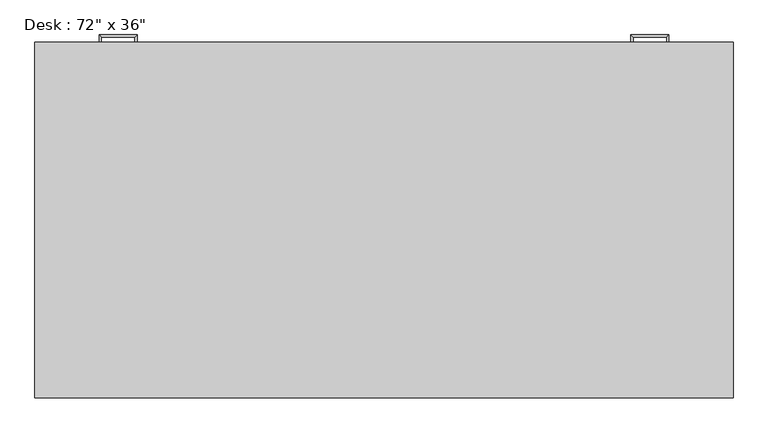
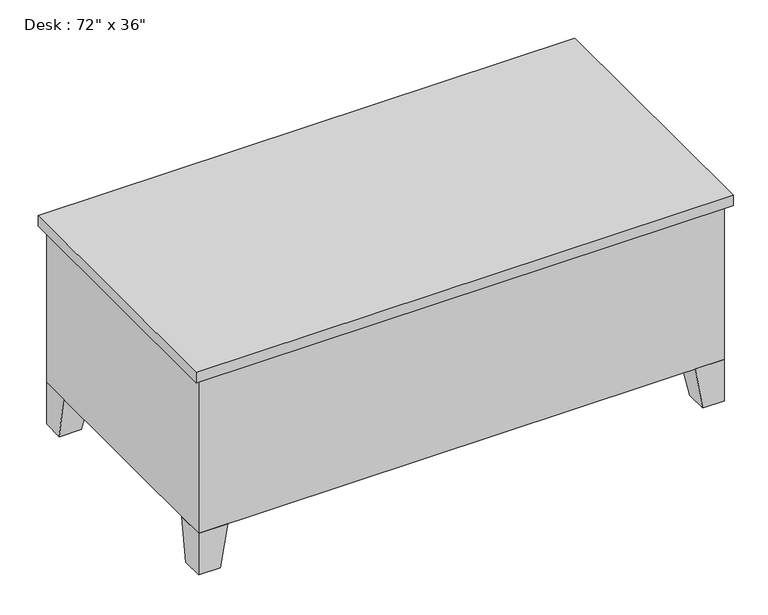
"""IFC4 building model written with IfcOpenShell, lengths in millimetres: furniture geometry."""

import ifcopenshell
import ifcopenshell.guid

model = None  # the IFC model being written
_history = None  # IfcOwnerHistory: only IFC2X3 demands one
_inside = {}  # id of a spatial element -> (the spatial element, [elements in it])
_under = {}  # id of a project, library or spatial element -> (it, [spatial elements below it])
_declared = {}  # id of a project -> (the project, [libraries it declares])
_typed = {}  # id of a type object -> (the type object, [elements of that type])
_made_of = {}  # id of a material, layer set ... -> (it, [elements and type objects made of it])


def new_model(schema):
    """Start an empty IFC model of exactly this schema.

    Asked for "IFC4X3", IfcOpenShell would pick the latest addendum, in which some entities
    have other attributes; the version numbers below select the first issue.
    IFC2X3 requires an IfcOwnerHistory on every rooted entity: one is made here for all.
    """
    global model, _history
    if schema == "IFC4X3":
        model = ifcopenshell.file(schema_version=(4, 3, 0, 0))
    else:
        model = ifcopenshell.file(schema=schema)
    _inside.clear()
    _under.clear()
    _declared.clear()
    _typed.clear()
    _made_of.clear()
    _history = None
    if model.schema == "IFC2X3":
        org = make("IfcOrganization", Name="unknown")
        user = make(
            "IfcPersonAndOrganization",
            ThePerson=make("IfcPerson", FamilyName="unknown"),
            TheOrganization=org,
        )
        app = make(
            "IfcApplication",
            ApplicationDeveloper=org,
            Version="unknown",
            ApplicationFullName="unknown",
            ApplicationIdentifier="unknown",
        )
        _history = make(
            "IfcOwnerHistory",
            OwningUser=user,
            OwningApplication=app,
            ChangeAction="ADDED",
            CreationDate=0,
        )
    return model


def make(cls, **values):
    """One entity of the class cls with the attributes given. An attribute that is None is left unset."""
    return model.create_entity(
        cls, **{name: value for name, value in values.items() if value is not None}
    )


def rooted(cls, **values):
    """An entity with a GlobalId (a new one), such as an element, a storey or a relation."""
    return make(cls, GlobalId=ifcopenshell.guid.new(), OwnerHistory=_history, **values)


def si_unit(unit_type, name, prefix=None):
    """IfcSIUnit, for example si_unit("LENGTHUNIT", "METRE", prefix="MILLI")."""
    return make("IfcSIUnit", UnitType=unit_type, Prefix=prefix, Name=name)


def assignment(units):
    """IfcUnitAssignment: the units of a project."""
    return None if units is None else make("IfcUnitAssignment", Units=units)


def point(xyz):
    """IfcCartesianPoint."""
    return None if xyz is None else make("IfcCartesianPoint", Coordinates=xyz)


def direction(xyz):
    """IfcDirection."""
    return None if xyz is None else make("IfcDirection", DirectionRatios=xyz)


def frame(location, z_axis=None, x_axis=None):
    """IfcAxis2Placement3D, a coordinate frame: its origin and axes. An axis left out is left unset."""
    return make(
        "IfcAxis2Placement3D",
        Location=point(location),
        Axis=direction(z_axis),
        RefDirection=direction(x_axis),
    )


def origin():
    """The frame at (0, 0, 0) with its axes left unset."""
    return frame((0.0, 0.0, 0.0))


def place(relative_to, where):
    """IfcLocalPlacement: puts the frame where relative to a parent placement (None: the world)."""
    return make(
        "IfcLocalPlacement", PlacementRelTo=relative_to, RelativePlacement=where
    )


def context(
    kind, dimensions, precision=None, world=None, true_north=None, identifier=None
):
    """IfcGeometricRepresentationContext, for example the 3D "Model" context."""
    return make(
        "IfcGeometricRepresentationContext",
        ContextIdentifier=identifier,
        ContextType=kind,
        CoordinateSpaceDimension=dimensions,
        Precision=precision,
        WorldCoordinateSystem=world,
        TrueNorth=true_north,
    )


def project(units=None, contexts=None):
    """IfcProject with its units and contexts."""
    return rooted(
        "IfcProject",
        Name="project",
        RepresentationContexts=contexts,
        UnitsInContext=assignment(units),
    )


def spatial(cls, under=None, at=None, **own):
    """A site, building, storey or space (cls), placed at a placement, below another one or the project."""
    s = rooted(cls, ObjectPlacement=at, **own)
    if under is not None:
        _under.setdefault(under.id(), (under, []))[1].append(s)
    return s


def polyline(points):
    """IfcPolyline through the points."""
    return make("IfcPolyline", Points=[point(p) for p in points])


def outline(outer, holes=None, kind="AREA"):
    """IfcArbitraryClosedProfileDef: a profile drawn as a closed curve; with holes, ...WithVoids."""
    if holes is None:
        return make("IfcArbitraryClosedProfileDef", ProfileType=kind, OuterCurve=outer)
    return make(
        "IfcArbitraryProfileDefWithVoids",
        ProfileType=kind,
        OuterCurve=outer,
        InnerCurves=holes,
    )


def extrude(swept, where, along, depth):
    """IfcExtrudedAreaSolid: the profile swept, set in the frame where, extruded along a direction by depth."""
    return make(
        "IfcExtrudedAreaSolid",
        SweptArea=swept,
        Position=where,
        ExtrudedDirection=direction(along),
        Depth=depth,
    )


def faces_of(points, faces, orient=None, outer=None):
    """IfcFace entities. A face is a list of loops; a loop is a list of indices into points, from 0.

    orient and outer hold one flag for each loop. By default every Orientation is true, the
    first loop of a face is its IfcFaceOuterBound and the others are IfcFaceBound.
    """
    made = []
    for i, loops in enumerate(faces):
        bounds = []
        for j, loop in enumerate(loops):
            is_outer = j == 0 if outer is None else outer[i][j]
            bounds.append(
                make(
                    "IfcFaceOuterBound" if is_outer else "IfcFaceBound",
                    Bound=make("IfcPolyLoop", Polygon=[points[k] for k in loop]),
                    Orientation=True if orient is None else orient[i][j],
                )
            )
        made.append(make("IfcFace", Bounds=bounds))
    return made


def faceted_brep(points, faces, orient=None, outer=None, voids=None):
    """IfcFacetedBrep: a solid bounded by flat faces; with voids (closed shells), ...WithVoids."""
    shared = [point(p) for p in points]
    hull = make("IfcClosedShell", CfsFaces=faces_of(shared, faces, orient, outer))
    if voids is None:
        return make("IfcFacetedBrep", Outer=hull)
    return make(
        "IfcFacetedBrepWithVoids",
        Outer=hull,
        Voids=[
            make(cls, CfsFaces=faces_of(shared, fs, o, b)) for cls, fs, o, b in voids
        ],
    )


def shape(context_of_items, identifier, shape_type, items):
    """IfcShapeRepresentation: the items that make up one representation, for example the "Body"."""
    return make(
        "IfcShapeRepresentation",
        ContextOfItems=context_of_items,
        RepresentationIdentifier=identifier,
        RepresentationType=shape_type,
        Items=items,
    )


def source(mapping_origin, context_of_items, identifier, shape_type, items):
    """IfcRepresentationMap: a shape defined once, which mapped items show again and again."""
    return make(
        "IfcRepresentationMap",
        MappingOrigin=mapping_origin,
        MappedRepresentation=shape(context_of_items, identifier, shape_type, items),
    )


def transform(
    local_origin,
    x_axis=None,
    y_axis=None,
    z_axis=None,
    scale=None,
    scale2=None,
    scale3=None,
    uniform=True,
):
    """IfcCartesianTransformationOperator3D, or its non-uniform kind. x_axis, y_axis, z_axis: its Axis1, 2, 3."""
    if uniform:
        return make(
            "IfcCartesianTransformationOperator3D",
            Axis1=direction(x_axis),
            Axis2=direction(y_axis),
            LocalOrigin=point(local_origin),
            Scale=scale,
            Axis3=direction(z_axis),
        )
    return make(
        "IfcCartesianTransformationOperator3DnonUniform",
        Axis1=direction(x_axis),
        Axis2=direction(y_axis),
        LocalOrigin=point(local_origin),
        Scale=scale,
        Axis3=direction(z_axis),
        Scale2=scale2,
        Scale3=scale3,
    )


def mapped(mapping_source, mapping_target):
    """IfcMappedItem: shows the shape of a source again, moved by a transform."""
    return make(
        "IfcMappedItem", MappingSource=mapping_source, MappingTarget=mapping_target
    )


def made_of(thing, what):
    """Note that an element or type object is made of a material, layer set ...; save() writes the relation."""
    if what is not None:
        _made_of.setdefault(what.id(), (what, []))[1].append(thing)
    return thing


def element(
    cls,
    number,
    at=None,
    inside=None,
    cuts=None,
    type_object=None,
    material=None,
    context=None,
    identifier="Body",
    shape_type=None,
    held_by="IfcProductDefinitionShape",
    body=None,
    shapes=None,
    **own,
):
    """One element of the class cls, such as IfcWall. Its Tag is "e" and its number.

    at: its placement. inside: the storey or other place that contains it. cuts: it is an
    opening in that element (IfcRelVoidsElement). A single representation is given by context,
    identifier, shape_type and body (its items); several are given by shapes. held_by: the class
    of the entity that holds the representations. save() writes the other relations.
    """
    e = rooted(cls, Tag="e%d" % number, ObjectPlacement=at, **own)
    if body is not None:
        shapes = [shape(context, identifier, shape_type, body)]
    if shapes is not None:
        e.Representation = make(held_by, Representations=shapes)
    if inside is not None:
        _inside.setdefault(inside.id(), (inside, []))[1].append(e)
    if cuts is not None:
        rooted(
            "IfcRelVoidsElement", RelatingBuildingElement=cuts, RelatedOpeningElement=e
        )
    if type_object is not None:
        _typed.setdefault(type_object.id(), (type_object, []))[1].append(e)
    return made_of(e, material)


def aggregate(whole, parts):
    """IfcRelAggregates: a whole, such as a stair, and the parts it consists of."""
    return rooted("IfcRelAggregates", RelatingObject=whole, RelatedObjects=parts)


def save(model, path):
    """Write the relations noted so far, then the file.

    IfcRelAggregates (storeys below a building ...), IfcRelContainedInSpatialStructure (elements
    in a storey), IfcRelDefinesByType, IfcRelAssociatesMaterial and IfcRelDeclares: one each for
    every whole, place, type object, material and project.
    """
    for whole, parts in _under.values():
        aggregate(whole, parts)
    for where, things in _inside.values():
        rooted(
            "IfcRelContainedInSpatialStructure",
            RelatedElements=things,
            RelatingStructure=where,
        )
    for kind, things in _typed.values():
        rooted("IfcRelDefinesByType", RelatedObjects=things, RelatingType=kind)
    for what, things in _made_of.values():
        rooted("IfcRelAssociatesMaterial", RelatedObjects=things, RelatingMaterial=what)
    for by, libraries in _declared.values():
        rooted("IfcRelDeclares", RelatingContext=by, RelatedDefinitions=libraries)
    model.write(path)


def furniture_2fc54265(model_context):
    return source(origin(), model_context, "Body", "SolidModel", [
        extrude(outline(polyline([(1809.75, 914.4), (1441.45, 914.4), (1441.45, 927.1), (1809.75, 927.1), (1809.75, 914.4)])), frame((0.0, 0.0, 603.25), z_axis=(0.0, 0.0, 1.0), x_axis=(1.0, 0.0, 0.0)), (0.0, 0.0, 1.0), 101.6),
        extrude(outline(polyline([(1809.75, 914.4), (1441.45, 914.4), (1441.45, 927.1), (1809.75, 927.1), (1809.75, 914.4)])), frame((0.0, 0.0, 171.45), z_axis=(0.0, 0.0, 1.0), x_axis=(1.0, 0.0, 0.0)), (0.0, 0.0, 1.0), 412.75),
        extrude(outline(polyline([(387.35, 914.4), (19.05, 914.4), (19.05, 927.1), (387.35, 927.1), (387.35, 914.4)])), frame((0.0, 0.0, 603.25), z_axis=(0.0, 0.0, 1.0), x_axis=(1.0, 0.0, 0.0)), (0.0, 0.0, 1.0), 101.6),
        extrude(outline(polyline([(387.35, 914.4), (19.05, 914.4), (19.05, 927.1), (387.35, 927.1), (387.35, 914.4)])), frame((0.0, 0.0, 171.45), z_axis=(0.0, 0.0, 1.0), x_axis=(1.0, 0.0, 0.0)), (0.0, 0.0, 1.0), 171.45),
        extrude(outline(polyline([(387.35, 914.4), (19.05, 914.4), (19.05, 927.1), (387.35, 927.1), (387.35, 914.4)])), frame((0.0, 0.0, 482.6), z_axis=(0.0, 0.0, 1.0), x_axis=(1.0, 0.0, 0.0)), (0.0, 0.0, 1.0), 101.6),
        extrude(outline(polyline([(387.35, 914.4), (19.05, 914.4), (19.05, 927.1), (387.35, 927.1), (387.35, 914.4)])), frame((0.0, 0.0, 361.95), z_axis=(0.0, 0.0, 1.0), x_axis=(1.0, 0.0, 0.0)), (0.0, 0.0, 1.0), 101.6),
        faceted_brep([(1727.2, 914.4, 152.4), (1727.2, 812.8, 152.4), (1828.8, 812.8, 152.4), (1828.8, 914.4, 152.4), (1752.6, 914.4, 0.0), (1828.8, 914.4, 0.0), (1828.8, 838.2, 0.0), (1752.6, 838.2, 0.0)], [[[0, 1, 2, 3]], [[4, 5, 6, 7]], [[4, 7, 1, 0]], [[7, 6, 2, 1]], [[6, 5, 3, 2]], [[5, 4, 0, 3]]]),
        faceted_brep([(1727.2, 0.0, 152.4), (1828.8, 0.0, 152.4), (1828.8, 101.6, 152.4), (1727.2, 101.6, 152.4), (1752.6, 0.0, 0.0), (1752.6, 76.2, 0.0), (1828.8, 76.2, 0.0), (1828.8, 0.0, 0.0)], [[[0, 1, 2, 3]], [[4, 5, 6, 7]], [[4, 7, 1, 0]], [[7, 6, 2, 1]], [[6, 5, 3, 2]], [[5, 4, 0, 3]]]),
        faceted_brep([(101.6, 0.0, 152.4), (101.6, 101.6, 152.4), (0.0, 101.6, 152.4), (0.0, 0.0, 152.4), (76.2, 0.0, 0.0), (0.0, 0.0, 0.0), (0.0, 76.2, 0.0), (76.2, 76.2, 0.0)], [[[0, 1, 2, 3]], [[4, 5, 6, 7]], [[4, 7, 1, 0]], [[7, 6, 2, 1]], [[6, 5, 3, 2]], [[5, 4, 0, 3]]]),
        faceted_brep([(101.6, 914.4, 152.4), (0.0, 914.4, 152.4), (0.0, 812.8, 152.4), (101.6, 812.8, 152.4), (76.2, 914.4, 0.0), (76.2, 838.2, 0.0), (0.0, 838.2, 0.0), (0.0, 914.4, 0.0)], [[[0, 1, 2, 3]], [[4, 5, 6, 7]], [[4, 7, 1, 0]], [[7, 6, 2, 1]], [[6, 5, 3, 2]], [[5, 4, 0, 3]]]),
        extrude(outline(polyline([(1847.85, 933.45), (1847.85, -19.05), (-19.05, -19.05), (-19.05, 933.45), (1847.85, 933.45)])), frame((0.0, 0.0, 723.9), z_axis=(0.0, 0.0, 1.0), x_axis=(1.0, 0.0, 0.0)), (0.0, 0.0, 1.0), 38.1),
        extrude(outline(polyline([(406.4, 914.4), (406.4, 50.8), (1422.4, 50.8), (1422.4, 914.4), (1828.8, 914.4), (1828.8, 0.0), (0.0, 0.0), (0.0, 914.4), (406.4, 914.4)])), frame((0.0, 0.0, 152.4), z_axis=(0.0, 0.0, 1.0), x_axis=(1.0, 0.0, 0.0)), (0.0, 0.0, 1.0), 571.5),
        faceted_brep([(1670.05, 927.1, 546.1), (1670.05, 927.1, 533.4), (1676.4, 927.1, 533.4), (1676.4, 927.1, 546.1), (1670.05, 946.15, 546.1), (1670.05, 946.15, 533.4), (1676.4, 952.5, 533.4), (1676.4, 952.5, 546.1), (1581.15, 946.15, 546.1), (1581.15, 946.15, 533.4), (1574.8, 952.5, 533.4), (1574.8, 952.5, 546.1), (1581.15, 927.1, 546.1), (1574.8, 927.1, 546.1), (1574.8, 927.1, 533.4), (1581.15, 927.1, 533.4)], [[[0, 1, 2, 3]], [[1, 0, 4, 5]], [[2, 1, 5, 6]], [[3, 2, 6, 7]], [[0, 3, 7, 4]], [[5, 4, 8, 9]], [[6, 5, 9, 10]], [[7, 6, 10, 11]], [[4, 7, 11, 8]], [[12, 13, 14, 15]], [[9, 8, 12, 15]], [[10, 9, 15, 14]], [[11, 10, 14, 13]], [[8, 11, 13, 12]]]),
        faceted_brep([(1670.05, 927.1, 666.75), (1670.05, 927.1, 654.05), (1676.4, 927.1, 654.05), (1676.4, 927.1, 666.75), (1670.05, 946.15, 666.75), (1670.05, 946.15, 654.05), (1676.4, 952.5, 654.05), (1676.4, 952.5, 666.75), (1581.15, 946.15, 666.75), (1581.15, 946.15, 654.05), (1574.8, 952.5, 654.05), (1574.8, 952.5, 666.75), (1581.15, 927.1, 666.75), (1574.8, 927.1, 666.75), (1574.8, 927.1, 654.05), (1581.15, 927.1, 654.05)], [[[0, 1, 2, 3]], [[1, 0, 4, 5]], [[2, 1, 5, 6]], [[3, 2, 6, 7]], [[0, 3, 7, 4]], [[5, 4, 8, 9]], [[6, 5, 9, 10]], [[7, 6, 10, 11]], [[4, 7, 11, 8]], [[12, 13, 14, 15]], [[9, 8, 12, 15]], [[10, 9, 15, 14]], [[11, 10, 14, 13]], [[8, 11, 13, 12]]]),
        faceted_brep([(158.75, 927.1, 304.8), (152.4, 927.1, 304.8), (152.4, 927.1, 292.1), (158.75, 927.1, 292.1), (158.75, 946.15, 304.8), (152.4, 952.5, 304.8), (152.4, 952.5, 292.1), (158.75, 946.15, 292.1), (247.65, 946.15, 304.8), (254.0, 952.5, 304.8), (254.0, 952.5, 292.1), (247.65, 946.15, 292.1), (247.65, 927.1, 304.8), (247.65, 927.1, 292.1), (254.0, 927.1, 292.1), (254.0, 927.1, 304.8)], [[[0, 1, 2, 3]], [[1, 0, 4, 5]], [[2, 1, 5, 6]], [[3, 2, 6, 7]], [[0, 3, 7, 4]], [[5, 4, 8, 9]], [[6, 5, 9, 10]], [[7, 6, 10, 11]], [[4, 7, 11, 8]], [[12, 13, 14, 15]], [[9, 8, 12, 15]], [[10, 9, 15, 14]], [[11, 10, 14, 13]], [[8, 11, 13, 12]]]),
        faceted_brep([(158.75, 927.1, 425.45), (152.4, 927.1, 425.45), (152.4, 927.1, 412.75), (158.75, 927.1, 412.75), (158.75, 946.15, 425.45), (152.4, 952.5, 425.45), (152.4, 952.5, 412.75), (158.75, 946.15, 412.75), (247.65, 946.15, 425.45), (254.0, 952.5, 425.45), (254.0, 952.5, 412.75), (247.65, 946.15, 412.75), (247.65, 927.1, 425.45), (247.65, 927.1, 412.75), (254.0, 927.1, 412.75), (254.0, 927.1, 425.45)], [[[0, 1, 2, 3]], [[1, 0, 4, 5]], [[2, 1, 5, 6]], [[3, 2, 6, 7]], [[0, 3, 7, 4]], [[5, 4, 8, 9]], [[6, 5, 9, 10]], [[7, 6, 10, 11]], [[4, 7, 11, 8]], [[12, 13, 14, 15]], [[9, 8, 12, 15]], [[10, 9, 15, 14]], [[11, 10, 14, 13]], [[8, 11, 13, 12]]]),
        faceted_brep([(158.75, 927.1, 546.1), (152.4, 927.1, 546.1), (152.4, 927.1, 533.4), (158.75, 927.1, 533.4), (158.75, 946.15, 546.1), (152.4, 952.5, 546.1), (152.4, 952.5, 533.4), (158.75, 946.15, 533.4), (247.65, 946.15, 546.1), (254.0, 952.5, 546.1), (254.0, 952.5, 533.4), (247.65, 946.15, 533.4), (247.65, 927.1, 546.1), (247.65, 927.1, 533.4), (254.0, 927.1, 533.4), (254.0, 927.1, 546.1)], [[[0, 1, 2, 3]], [[1, 0, 4, 5]], [[2, 1, 5, 6]], [[3, 2, 6, 7]], [[0, 3, 7, 4]], [[5, 4, 8, 9]], [[6, 5, 9, 10]], [[7, 6, 10, 11]], [[4, 7, 11, 8]], [[12, 13, 14, 15]], [[9, 8, 12, 15]], [[10, 9, 15, 14]], [[11, 10, 14, 13]], [[8, 11, 13, 12]]]),
        faceted_brep([(158.75, 927.1, 666.75), (152.4, 927.1, 666.75), (152.4, 927.1, 654.05), (158.75, 927.1, 654.05), (158.75, 946.15, 666.75), (152.4, 952.5, 666.75), (152.4, 952.5, 654.05), (158.75, 946.15, 654.05), (247.65, 946.15, 666.75), (254.0, 952.5, 666.75), (254.0, 952.5, 654.05), (247.65, 946.15, 654.05), (247.65, 927.1, 666.75), (247.65, 927.1, 654.05), (254.0, 927.1, 654.05), (254.0, 927.1, 666.75)], [[[0, 1, 2, 3]], [[1, 0, 4, 5]], [[2, 1, 5, 6]], [[3, 2, 6, 7]], [[0, 3, 7, 4]], [[5, 4, 8, 9]], [[6, 5, 9, 10]], [[7, 6, 10, 11]], [[4, 7, 11, 8]], [[12, 13, 14, 15]], [[9, 8, 12, 15]], [[10, 9, 15, 14]], [[11, 10, 14, 13]], [[8, 11, 13, 12]]]),
    ])


if __name__ == "__main__":
    model = new_model("IFC4")
    model_context = context("Model", 3, world=origin())
    ifc_project = project(units=[si_unit("LENGTHUNIT", "METRE", prefix="MILLI")], contexts=[model_context])
    site = spatial("IfcSite", under=ifc_project)
    building = spatial("IfcBuilding", under=site)
    placement = place(None, origin())
    furniture_shape = furniture_2fc54265(model_context)
    element("IfcFurniture", 1, ObjectType="Desk : 72\" x 36\"", at=placement, inside=building, context=model_context, shape_type="MappedRepresentation", body=[
        mapped(furniture_shape, transform((0.0, 0.0, 0.0), x_axis=(1.0, 0.0, 0.0), y_axis=(0.0, 1.0, 0.0), z_axis=(0.0, 0.0, 1.0))),
    ])
    save(model, "model.ifc")

# Revit data of these elements
# Type "Desk : 72\" x 36\""
#   Assembly Code = "E2020200"
#   Depth = 3' - 0"
#   Height = 2' - 6"
#   Leg Height = 0' - 6"
#   Width = 6' - 0"
#   Body Material = Laminate, Ivory, Matte
#   Handle/Leg Material = Steel, Chrome Plated
#   Top Material = Cherry
#   Default Elevation = 0
# Element 1 (IfcFurniture, "Desk : 72\" x 36\"")
#   Materials on its faces: "Steel, Chrome Plated", "Laminate, Ivory, Matte", "Cherry"
# Materials
#   "Laminate, Ivory, Matte": class "Plastic", colour RGB 247 247 239, transparency 0, Description = "Plastic Laminate - Ivory, Matte", Cost = 0
#   "Steel, Chrome Plated": class "Metal", colour RGB 17 17 17, transparency 0, Description = "Chromiuim plated steel", Cost = 0
#   "Cherry": class "Wood", colour RGB 226 177 128, transparency 0, Description = "Prunus Serotina", Cost = 0
